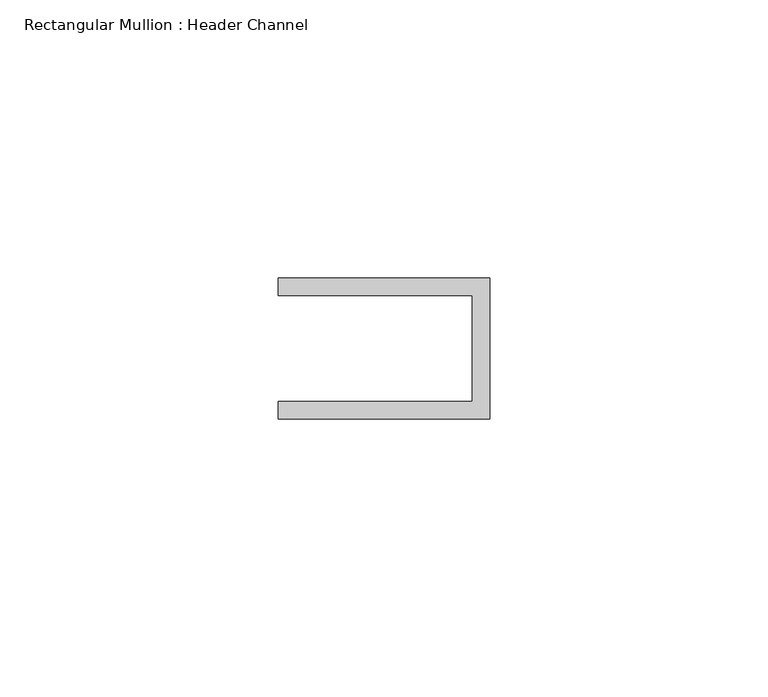
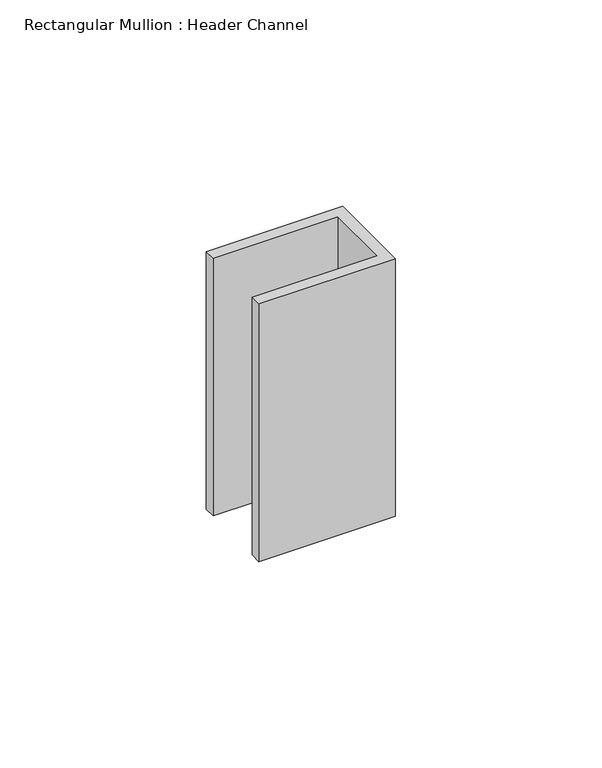
"""IFC4 building model written with IfcOpenShell, lengths in millimetres: member geometry, Rectangular Mullion : Header Channel."""

from ifc_helpers import new_model, si_unit, frame, origin, place, context, project, spatial, polyline, outline, extrude, source, transform, mapped, element, save


def rectangular_mullion_header_channel_f14c0fb3(model_context):
    return source(origin(), model_context, "Body", "SweptSolid", [
        extrude(outline(polyline([(0.0, 12.7), (0.0, -12.7), (-38.1, -12.7), (-38.1, -9.525), (-3.175, -9.525), (-3.175, 9.525), (-38.1, 9.525), (-38.1, 12.7), (0.0, 12.7)])), frame((0.0, 0.0, -76.2), z_axis=(0.0, 0.0, 1.0), x_axis=(1.0, 0.0, 0.0)), (0.0, 0.0, 1.0), 76.2),
    ])


if __name__ == "__main__":
    model = new_model("IFC4")
    model_context = context("Model", 3, world=origin())
    ifc_project = project(units=[si_unit("LENGTHUNIT", "METRE", prefix="MILLI")], contexts=[model_context])
    site = spatial("IfcSite", under=ifc_project)
    building = spatial("IfcBuilding", under=site)
    placement = place(None, origin())
    rectangular_mullion_header_channel_shape = rectangular_mullion_header_channel_f14c0fb3(model_context)
    element("IfcMember", 1, ObjectType="Rectangular Mullion : Header Channel", at=placement, inside=building, context=model_context, shape_type="MappedRepresentation", body=[
        mapped(rectangular_mullion_header_channel_shape, transform((0.0, 0.0, 0.0), x_axis=(1.0, 0.0, 0.0), y_axis=(0.0, 1.0, 0.0), z_axis=(0.0, 0.0, 1.0))),
    ])
    save(model, "model.ifc")

# Revit data of these elements
# Type "Rectangular Mullion : Header Channel"
#   built-in parameter 1007322 = 0.0833333 (stored number, unit not read)
#   built-in parameter 1007321 = -0.03125 (stored number, unit not read)
#   built-in parameter 1007320 = 0.0416667 (stored number, unit not read)
# Element 1 (IfcMember, "Rectangular Mullion : Header Channel")
#   Materials on its faces: "ALUM"
# Materials
#   "ALUM": class "Generic", colour RGB 157 157 157, transparency 0, Cost = 0
